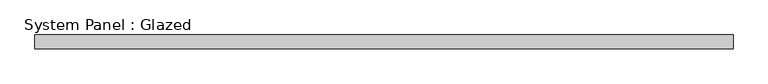
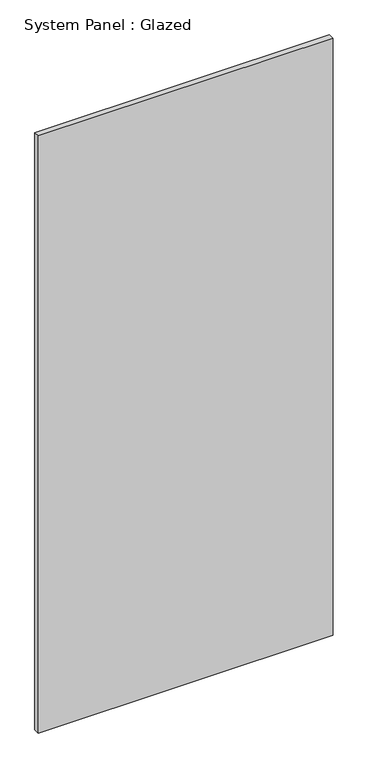
"""IFC4 building model written with IfcOpenShell, lengths in millimetres: plate geometry, System Panel : Glazed."""

import ifcopenshell
import ifcopenshell.guid

model = None  # the IFC model being written
_history = None  # IfcOwnerHistory: only IFC2X3 demands one
_inside = {}  # id of a spatial element -> (the spatial element, [elements in it])
_under = {}  # id of a project, library or spatial element -> (it, [spatial elements below it])
_declared = {}  # id of a project -> (the project, [libraries it declares])
_typed = {}  # id of a type object -> (the type object, [elements of that type])
_made_of = {}  # id of a material, layer set ... -> (it, [elements and type objects made of it])


def new_model(schema):
    """Start an empty IFC model of exactly this schema.

    Asked for "IFC4X3", IfcOpenShell would pick the latest addendum, in which some entities
    have other attributes; the version numbers below select the first issue.
    IFC2X3 requires an IfcOwnerHistory on every rooted entity: one is made here for all.
    """
    global model, _history
    if schema == "IFC4X3":
        model = ifcopenshell.file(schema_version=(4, 3, 0, 0))
    else:
        model = ifcopenshell.file(schema=schema)
    _inside.clear()
    _under.clear()
    _declared.clear()
    _typed.clear()
    _made_of.clear()
    _history = None
    if model.schema == "IFC2X3":
        org = make("IfcOrganization", Name="unknown")
        user = make(
            "IfcPersonAndOrganization",
            ThePerson=make("IfcPerson", FamilyName="unknown"),
            TheOrganization=org,
        )
        app = make(
            "IfcApplication",
            ApplicationDeveloper=org,
            Version="unknown",
            ApplicationFullName="unknown",
            ApplicationIdentifier="unknown",
        )
        _history = make(
            "IfcOwnerHistory",
            OwningUser=user,
            OwningApplication=app,
            ChangeAction="ADDED",
            CreationDate=0,
        )
    return model


def make(cls, **values):
    """One entity of the class cls with the attributes given. An attribute that is None is left unset."""
    return model.create_entity(
        cls, **{name: value for name, value in values.items() if value is not None}
    )


def rooted(cls, **values):
    """An entity with a GlobalId (a new one), such as an element, a storey or a relation."""
    return make(cls, GlobalId=ifcopenshell.guid.new(), OwnerHistory=_history, **values)


def si_unit(unit_type, name, prefix=None):
    """IfcSIUnit, for example si_unit("LENGTHUNIT", "METRE", prefix="MILLI")."""
    return make("IfcSIUnit", UnitType=unit_type, Prefix=prefix, Name=name)


def assignment(units):
    """IfcUnitAssignment: the units of a project."""
    return None if units is None else make("IfcUnitAssignment", Units=units)


def point(xyz):
    """IfcCartesianPoint."""
    return None if xyz is None else make("IfcCartesianPoint", Coordinates=xyz)


def direction(xyz):
    """IfcDirection."""
    return None if xyz is None else make("IfcDirection", DirectionRatios=xyz)


def frame(location, z_axis=None, x_axis=None):
    """IfcAxis2Placement3D, a coordinate frame: its origin and axes. An axis left out is left unset."""
    return make(
        "IfcAxis2Placement3D",
        Location=point(location),
        Axis=direction(z_axis),
        RefDirection=direction(x_axis),
    )


def origin():
    """The frame at (0, 0, 0) with its axes left unset."""
    return frame((0.0, 0.0, 0.0))


def origin_with_axes():
    """The frame at (0, 0, 0) with the z axis (0, 0, 1) and the x axis (1, 0, 0) written out."""
    return frame((0.0, 0.0, 0.0), z_axis=(0.0, 0.0, 1.0), x_axis=(1.0, 0.0, 0.0))


def place(relative_to, where):
    """IfcLocalPlacement: puts the frame where relative to a parent placement (None: the world)."""
    return make(
        "IfcLocalPlacement", PlacementRelTo=relative_to, RelativePlacement=where
    )


def context(
    kind, dimensions, precision=None, world=None, true_north=None, identifier=None
):
    """IfcGeometricRepresentationContext, for example the 3D "Model" context."""
    return make(
        "IfcGeometricRepresentationContext",
        ContextIdentifier=identifier,
        ContextType=kind,
        CoordinateSpaceDimension=dimensions,
        Precision=precision,
        WorldCoordinateSystem=world,
        TrueNorth=true_north,
    )


def project(units=None, contexts=None):
    """IfcProject with its units and contexts."""
    return rooted(
        "IfcProject",
        Name="project",
        RepresentationContexts=contexts,
        UnitsInContext=assignment(units),
    )


def spatial(cls, under=None, at=None, **own):
    """A site, building, storey or space (cls), placed at a placement, below another one or the project."""
    s = rooted(cls, ObjectPlacement=at, **own)
    if under is not None:
        _under.setdefault(under.id(), (under, []))[1].append(s)
    return s


def polyline(points):
    """IfcPolyline through the points."""
    return make("IfcPolyline", Points=[point(p) for p in points])


def outline(outer, holes=None, kind="AREA"):
    """IfcArbitraryClosedProfileDef: a profile drawn as a closed curve; with holes, ...WithVoids."""
    if holes is None:
        return make("IfcArbitraryClosedProfileDef", ProfileType=kind, OuterCurve=outer)
    return make(
        "IfcArbitraryProfileDefWithVoids",
        ProfileType=kind,
        OuterCurve=outer,
        InnerCurves=holes,
    )


def extrude(swept, where, along, depth):
    """IfcExtrudedAreaSolid: the profile swept, set in the frame where, extruded along a direction by depth."""
    return make(
        "IfcExtrudedAreaSolid",
        SweptArea=swept,
        Position=where,
        ExtrudedDirection=direction(along),
        Depth=depth,
    )


def shape(context_of_items, identifier, shape_type, items):
    """IfcShapeRepresentation: the items that make up one representation, for example the "Body"."""
    return make(
        "IfcShapeRepresentation",
        ContextOfItems=context_of_items,
        RepresentationIdentifier=identifier,
        RepresentationType=shape_type,
        Items=items,
    )


def source(mapping_origin, context_of_items, identifier, shape_type, items):
    """IfcRepresentationMap: a shape defined once, which mapped items show again and again."""
    return make(
        "IfcRepresentationMap",
        MappingOrigin=mapping_origin,
        MappedRepresentation=shape(context_of_items, identifier, shape_type, items),
    )


def transform(
    local_origin,
    x_axis=None,
    y_axis=None,
    z_axis=None,
    scale=None,
    scale2=None,
    scale3=None,
    uniform=True,
):
    """IfcCartesianTransformationOperator3D, or its non-uniform kind. x_axis, y_axis, z_axis: its Axis1, 2, 3."""
    if uniform:
        return make(
            "IfcCartesianTransformationOperator3D",
            Axis1=direction(x_axis),
            Axis2=direction(y_axis),
            LocalOrigin=point(local_origin),
            Scale=scale,
            Axis3=direction(z_axis),
        )
    return make(
        "IfcCartesianTransformationOperator3DnonUniform",
        Axis1=direction(x_axis),
        Axis2=direction(y_axis),
        LocalOrigin=point(local_origin),
        Scale=scale,
        Axis3=direction(z_axis),
        Scale2=scale2,
        Scale3=scale3,
    )


def mapped(mapping_source, mapping_target):
    """IfcMappedItem: shows the shape of a source again, moved by a transform."""
    return make(
        "IfcMappedItem", MappingSource=mapping_source, MappingTarget=mapping_target
    )


def made_of(thing, what):
    """Note that an element or type object is made of a material, layer set ...; save() writes the relation."""
    if what is not None:
        _made_of.setdefault(what.id(), (what, []))[1].append(thing)
    return thing


def element(
    cls,
    number,
    at=None,
    inside=None,
    cuts=None,
    type_object=None,
    material=None,
    context=None,
    identifier="Body",
    shape_type=None,
    held_by="IfcProductDefinitionShape",
    body=None,
    shapes=None,
    **own,
):
    """One element of the class cls, such as IfcWall. Its Tag is "e" and its number.

    at: its placement. inside: the storey or other place that contains it. cuts: it is an
    opening in that element (IfcRelVoidsElement). A single representation is given by context,
    identifier, shape_type and body (its items); several are given by shapes. held_by: the class
    of the entity that holds the representations. save() writes the other relations.
    """
    e = rooted(cls, Tag="e%d" % number, ObjectPlacement=at, **own)
    if body is not None:
        shapes = [shape(context, identifier, shape_type, body)]
    if shapes is not None:
        e.Representation = make(held_by, Representations=shapes)
    if inside is not None:
        _inside.setdefault(inside.id(), (inside, []))[1].append(e)
    if cuts is not None:
        rooted(
            "IfcRelVoidsElement", RelatingBuildingElement=cuts, RelatedOpeningElement=e
        )
    if type_object is not None:
        _typed.setdefault(type_object.id(), (type_object, []))[1].append(e)
    return made_of(e, material)


def aggregate(whole, parts):
    """IfcRelAggregates: a whole, such as a stair, and the parts it consists of."""
    return rooted("IfcRelAggregates", RelatingObject=whole, RelatedObjects=parts)


def save(model, path):
    """Write the relations noted so far, then the file.

    IfcRelAggregates (storeys below a building ...), IfcRelContainedInSpatialStructure (elements
    in a storey), IfcRelDefinesByType, IfcRelAssociatesMaterial and IfcRelDeclares: one each for
    every whole, place, type object, material and project.
    """
    for whole, parts in _under.values():
        aggregate(whole, parts)
    for where, things in _inside.values():
        rooted(
            "IfcRelContainedInSpatialStructure",
            RelatedElements=things,
            RelatingStructure=where,
        )
    for kind, things in _typed.values():
        rooted("IfcRelDefinesByType", RelatedObjects=things, RelatingType=kind)
    for what, things in _made_of.values():
        rooted("IfcRelAssociatesMaterial", RelatedObjects=things, RelatingMaterial=what)
    for by, libraries in _declared.values():
        rooted("IfcRelDeclares", RelatingContext=by, RelatedDefinitions=libraries)
    model.write(path)


def system_panel_glazed_3a20483a(model_context):
    return source(origin(), model_context, "Body", "SweptSolid", [
        extrude(outline(polyline([(651.3841868, 19.05), (-651.3841868, 19.05), (-651.3841868, 44.45), (651.3841868, 44.45), (651.3841868, 19.05)])), origin_with_axes(), (0.0, 0.0, 1.0), 2788.92),
    ])


if __name__ == "__main__":
    model = new_model("IFC4")
    model_context = context("Model", 3, world=origin())
    ifc_project = project(units=[si_unit("LENGTHUNIT", "METRE", prefix="MILLI")], contexts=[model_context])
    site = spatial("IfcSite", under=ifc_project)
    building = spatial("IfcBuilding", under=site)
    placement = place(None, origin())
    system_panel_glazed_shape = system_panel_glazed_3a20483a(model_context)
    element("IfcPlate", 1, ObjectType="System Panel : Glazed", at=placement, inside=building, context=model_context, shape_type="MappedRepresentation", body=[
        mapped(system_panel_glazed_shape, transform((0.0, 0.0, 0.0), x_axis=(1.0, 0.0, 0.0), y_axis=(0.0, 1.0, 0.0), z_axis=(0.0, 0.0, 1.0))),
    ])
    save(model, "model.ifc")

# Revit data of these elements
# Type "System Panel : Glazed"
#   Construction Type Id = "GSP4R"
#   Analytic Construction = "1/8 in Pilkington single glazing"
#   Visual Light Transmittance = 0.9
#   Solar Heat Gain Coefficient = 0.86
#   Heat Transfer Coefficient (U) = 1.18115 BTU/(h·ft²·°F)
#   Define Thermal Properties by = 1
# Element 1 (IfcPlate, "System Panel : Glazed")
#   Materials on its faces: "Glass"
# Materials
#   "Glass": class "Glass", colour RGB 0 128 192, transparency 0.75, Description = "Soda Lime Glass", Cost = 0
